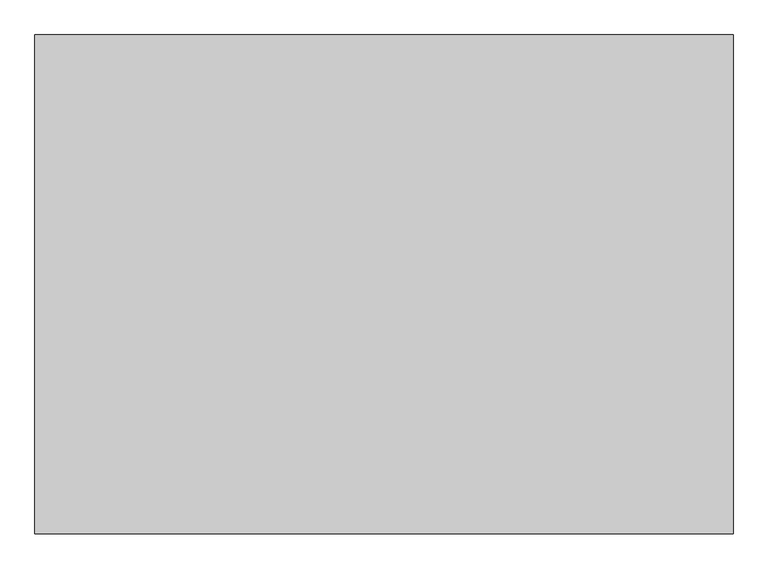
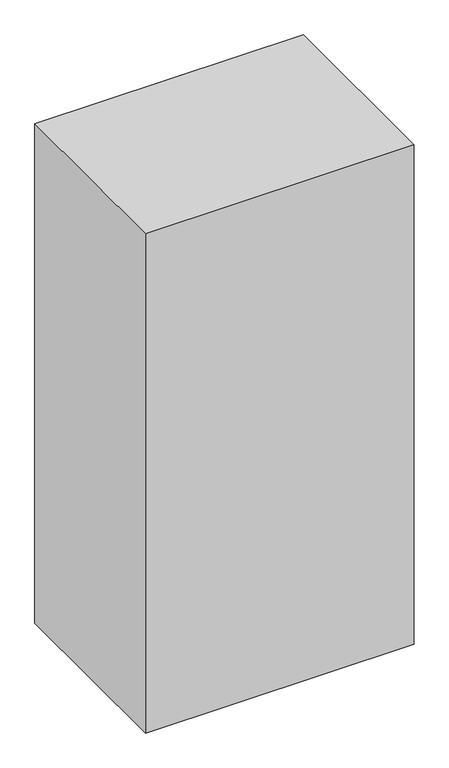
"""IFC4 building model written with IfcOpenShell, lengths in millimetres: proxy geometry, Space Planning Box_hec : Space Planning Box_hec."""

from ifc_helpers import new_model, si_unit, origin, origin_with_axes, place, context, project, spatial, polyline, outline, extrude, source, transform, mapped, element, save


def generic_models_ee32b0c6(model_context):
    return source(origin(), model_context, "Body", "SweptSolid", [
        extrude(outline(polyline([(1400.0, 1000.0), (1400.0, -1000.0), (-1400.0, -1000.0), (-1400.0, 1000.0), (1400.0, 1000.0)])), origin_with_axes(), (0.0, 0.0, 1.0), 5500.0),
    ])


if __name__ == "__main__":
    model = new_model("IFC4")
    model_context = context("Model", 3, world=origin())
    ifc_project = project(units=[si_unit("LENGTHUNIT", "METRE", prefix="MILLI")], contexts=[model_context])
    site = spatial("IfcSite", under=ifc_project)
    building = spatial("IfcBuilding", under=site)
    placement = place(None, origin())
    generic_models_shape = generic_models_ee32b0c6(model_context)
    element("IfcBuildingElementProxy", 1, Name="Space Planning Box_hec : Space Planning Box_hec", ObjectType="Space Planning Box_hec : Space Planning Box_hec", at=placement, inside=building, context=model_context, shape_type="MappedRepresentation", body=[
        mapped(generic_models_shape, transform((0.0, 0.0, 0.0), x_axis=(1.0, 0.0, 0.0), y_axis=(0.0, 1.0, 0.0), z_axis=(0.0, 0.0, 1.0))),
    ])
    save(model, "model.ifc")

# Revit data of these elements
# Type "Space Planning Box_hec : Space Planning Box_hec"
#   Type Comments = "..."
#   Room Name [instance default] = "?"
#   Interior Finish [instance default] = ""
#   Exterior Finish [instance default] = ""
#   Department [instance default] = ""
#   Assembly Code = "..."
#   ceiling height [instance default] = 0
#   Width [instance default] = 1524 mm
#   Program Area [instance default] = 0.00 m²
#   Length [instance default] = 1524 mm
#   Height [instance default] = 1524 mm
#   Area [instance default] = 2.32258 m²
#   Fill Color [instance default] = Cyan
#   Default Elevation = 0
# Element 1 (IfcBuildingElementProxy, "Space Planning Box_hec : Space Planning Box_hec")
#   Room Name = "Shower"
#   Exterior Finish = "N/A..N/A,,EW2..N/A..N/A"
#   Department = "AR"
#   Width = 2800 mm
#   Program Area = 5.60 m²
#   Length = 2000 mm
#   Height = 5500 mm
#   Area = 5.60 m²
#   Materials on its faces: "Cyan"
# Materials
#   "Cyan": class "Generic", colour RGB 0 255 255, transparency 0.2, Cost = 0
